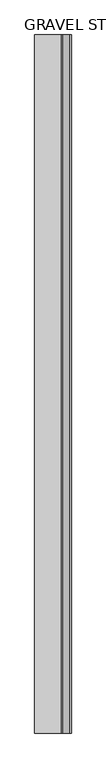
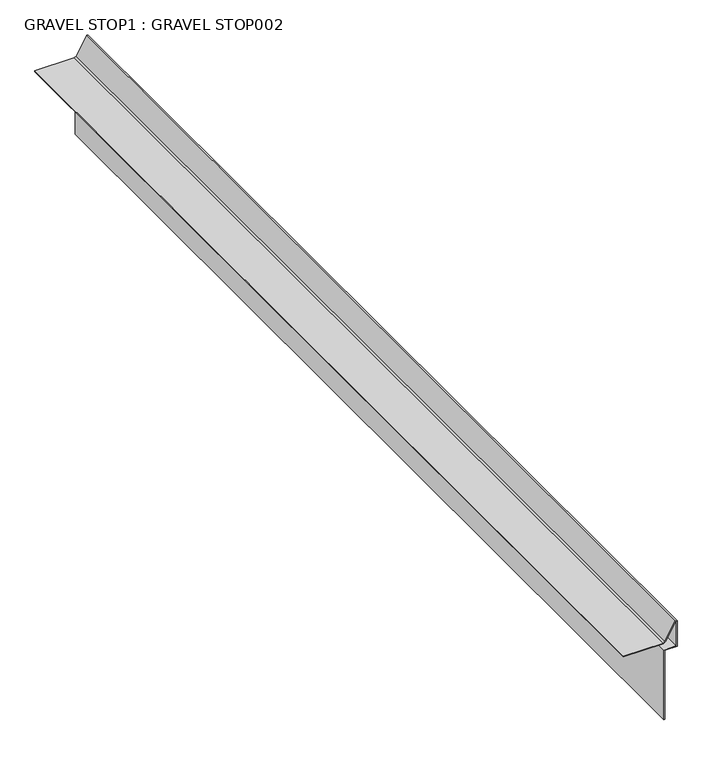
"""IFC4 building model written with IfcOpenShell, lengths in millimetres: proxy geometry, GRAVEL STOP1 : GRAVEL STOP002."""

import ifcopenshell
import ifcopenshell.guid

model = None  # the IFC model being written
_history = None  # IfcOwnerHistory: only IFC2X3 demands one
_inside = {}  # id of a spatial element -> (the spatial element, [elements in it])
_under = {}  # id of a project, library or spatial element -> (it, [spatial elements below it])
_declared = {}  # id of a project -> (the project, [libraries it declares])
_typed = {}  # id of a type object -> (the type object, [elements of that type])
_made_of = {}  # id of a material, layer set ... -> (it, [elements and type objects made of it])


def new_model(schema):
    """Start an empty IFC model of exactly this schema.

    Asked for "IFC4X3", IfcOpenShell would pick the latest addendum, in which some entities
    have other attributes; the version numbers below select the first issue.
    IFC2X3 requires an IfcOwnerHistory on every rooted entity: one is made here for all.
    """
    global model, _history
    if schema == "IFC4X3":
        model = ifcopenshell.file(schema_version=(4, 3, 0, 0))
    else:
        model = ifcopenshell.file(schema=schema)
    _inside.clear()
    _under.clear()
    _declared.clear()
    _typed.clear()
    _made_of.clear()
    _history = None
    if model.schema == "IFC2X3":
        org = make("IfcOrganization", Name="unknown")
        user = make(
            "IfcPersonAndOrganization",
            ThePerson=make("IfcPerson", FamilyName="unknown"),
            TheOrganization=org,
        )
        app = make(
            "IfcApplication",
            ApplicationDeveloper=org,
            Version="unknown",
            ApplicationFullName="unknown",
            ApplicationIdentifier="unknown",
        )
        _history = make(
            "IfcOwnerHistory",
            OwningUser=user,
            OwningApplication=app,
            ChangeAction="ADDED",
            CreationDate=0,
        )
    return model


def make(cls, **values):
    """One entity of the class cls with the attributes given. An attribute that is None is left unset."""
    return model.create_entity(
        cls, **{name: value for name, value in values.items() if value is not None}
    )


def rooted(cls, **values):
    """An entity with a GlobalId (a new one), such as an element, a storey or a relation."""
    return make(cls, GlobalId=ifcopenshell.guid.new(), OwnerHistory=_history, **values)


def si_unit(unit_type, name, prefix=None):
    """IfcSIUnit, for example si_unit("LENGTHUNIT", "METRE", prefix="MILLI")."""
    return make("IfcSIUnit", UnitType=unit_type, Prefix=prefix, Name=name)


def assignment(units):
    """IfcUnitAssignment: the units of a project."""
    return None if units is None else make("IfcUnitAssignment", Units=units)


def point(xyz):
    """IfcCartesianPoint."""
    return None if xyz is None else make("IfcCartesianPoint", Coordinates=xyz)


def direction(xyz):
    """IfcDirection."""
    return None if xyz is None else make("IfcDirection", DirectionRatios=xyz)


def frame(location, z_axis=None, x_axis=None):
    """IfcAxis2Placement3D, a coordinate frame: its origin and axes. An axis left out is left unset."""
    return make(
        "IfcAxis2Placement3D",
        Location=point(location),
        Axis=direction(z_axis),
        RefDirection=direction(x_axis),
    )


def origin():
    """The frame at (0, 0, 0) with its axes left unset."""
    return frame((0.0, 0.0, 0.0))


def place(relative_to, where):
    """IfcLocalPlacement: puts the frame where relative to a parent placement (None: the world)."""
    return make(
        "IfcLocalPlacement", PlacementRelTo=relative_to, RelativePlacement=where
    )


def context(
    kind, dimensions, precision=None, world=None, true_north=None, identifier=None
):
    """IfcGeometricRepresentationContext, for example the 3D "Model" context."""
    return make(
        "IfcGeometricRepresentationContext",
        ContextIdentifier=identifier,
        ContextType=kind,
        CoordinateSpaceDimension=dimensions,
        Precision=precision,
        WorldCoordinateSystem=world,
        TrueNorth=true_north,
    )


def project(units=None, contexts=None):
    """IfcProject with its units and contexts."""
    return rooted(
        "IfcProject",
        Name="project",
        RepresentationContexts=contexts,
        UnitsInContext=assignment(units),
    )


def spatial(cls, under=None, at=None, **own):
    """A site, building, storey or space (cls), placed at a placement, below another one or the project."""
    s = rooted(cls, ObjectPlacement=at, **own)
    if under is not None:
        _under.setdefault(under.id(), (under, []))[1].append(s)
    return s


def polyline(points):
    """IfcPolyline through the points."""
    return make("IfcPolyline", Points=[point(p) for p in points])


def outline(outer, holes=None, kind="AREA"):
    """IfcArbitraryClosedProfileDef: a profile drawn as a closed curve; with holes, ...WithVoids."""
    if holes is None:
        return make("IfcArbitraryClosedProfileDef", ProfileType=kind, OuterCurve=outer)
    return make(
        "IfcArbitraryProfileDefWithVoids",
        ProfileType=kind,
        OuterCurve=outer,
        InnerCurves=holes,
    )


def extrude(swept, where, along, depth):
    """IfcExtrudedAreaSolid: the profile swept, set in the frame where, extruded along a direction by depth."""
    return make(
        "IfcExtrudedAreaSolid",
        SweptArea=swept,
        Position=where,
        ExtrudedDirection=direction(along),
        Depth=depth,
    )


def shape(context_of_items, identifier, shape_type, items):
    """IfcShapeRepresentation: the items that make up one representation, for example the "Body"."""
    return make(
        "IfcShapeRepresentation",
        ContextOfItems=context_of_items,
        RepresentationIdentifier=identifier,
        RepresentationType=shape_type,
        Items=items,
    )


def source(mapping_origin, context_of_items, identifier, shape_type, items):
    """IfcRepresentationMap: a shape defined once, which mapped items show again and again."""
    return make(
        "IfcRepresentationMap",
        MappingOrigin=mapping_origin,
        MappedRepresentation=shape(context_of_items, identifier, shape_type, items),
    )


def transform(
    local_origin,
    x_axis=None,
    y_axis=None,
    z_axis=None,
    scale=None,
    scale2=None,
    scale3=None,
    uniform=True,
):
    """IfcCartesianTransformationOperator3D, or its non-uniform kind. x_axis, y_axis, z_axis: its Axis1, 2, 3."""
    if uniform:
        return make(
            "IfcCartesianTransformationOperator3D",
            Axis1=direction(x_axis),
            Axis2=direction(y_axis),
            LocalOrigin=point(local_origin),
            Scale=scale,
            Axis3=direction(z_axis),
        )
    return make(
        "IfcCartesianTransformationOperator3DnonUniform",
        Axis1=direction(x_axis),
        Axis2=direction(y_axis),
        LocalOrigin=point(local_origin),
        Scale=scale,
        Axis3=direction(z_axis),
        Scale2=scale2,
        Scale3=scale3,
    )


def mapped(mapping_source, mapping_target):
    """IfcMappedItem: shows the shape of a source again, moved by a transform."""
    return make(
        "IfcMappedItem", MappingSource=mapping_source, MappingTarget=mapping_target
    )


def made_of(thing, what):
    """Note that an element or type object is made of a material, layer set ...; save() writes the relation."""
    if what is not None:
        _made_of.setdefault(what.id(), (what, []))[1].append(thing)
    return thing


def element(
    cls,
    number,
    at=None,
    inside=None,
    cuts=None,
    type_object=None,
    material=None,
    context=None,
    identifier="Body",
    shape_type=None,
    held_by="IfcProductDefinitionShape",
    body=None,
    shapes=None,
    **own,
):
    """One element of the class cls, such as IfcWall. Its Tag is "e" and its number.

    at: its placement. inside: the storey or other place that contains it. cuts: it is an
    opening in that element (IfcRelVoidsElement). A single representation is given by context,
    identifier, shape_type and body (its items); several are given by shapes. held_by: the class
    of the entity that holds the representations. save() writes the other relations.
    """
    e = rooted(cls, Tag="e%d" % number, ObjectPlacement=at, **own)
    if body is not None:
        shapes = [shape(context, identifier, shape_type, body)]
    if shapes is not None:
        e.Representation = make(held_by, Representations=shapes)
    if inside is not None:
        _inside.setdefault(inside.id(), (inside, []))[1].append(e)
    if cuts is not None:
        rooted(
            "IfcRelVoidsElement", RelatingBuildingElement=cuts, RelatedOpeningElement=e
        )
    if type_object is not None:
        _typed.setdefault(type_object.id(), (type_object, []))[1].append(e)
    return made_of(e, material)


def aggregate(whole, parts):
    """IfcRelAggregates: a whole, such as a stair, and the parts it consists of."""
    return rooted("IfcRelAggregates", RelatingObject=whole, RelatedObjects=parts)


def save(model, path):
    """Write the relations noted so far, then the file.

    IfcRelAggregates (storeys below a building ...), IfcRelContainedInSpatialStructure (elements
    in a storey), IfcRelDefinesByType, IfcRelAssociatesMaterial and IfcRelDeclares: one each for
    every whole, place, type object, material and project.
    """
    for whole, parts in _under.values():
        aggregate(whole, parts)
    for where, things in _inside.values():
        rooted(
            "IfcRelContainedInSpatialStructure",
            RelatedElements=things,
            RelatingStructure=where,
        )
    for kind, things in _typed.values():
        rooted("IfcRelDefinesByType", RelatedObjects=things, RelatingType=kind)
    for what, things in _made_of.values():
        rooted("IfcRelAssociatesMaterial", RelatedObjects=things, RelatingMaterial=what)
    for by, libraries in _declared.values():
        rooted("IfcRelDeclares", RelatingContext=by, RelatedDefinitions=libraries)
    model.write(path)


def gravel_stop1_gravel_stop002_7041c615(model_context):
    return source(origin(), model_context, "Body", "SweptSolid", [
        extrude(outline(polyline([(40295.3431515, -4364.7039765), (40259.5408757, -4385.3744301), (40257.3744784, -4389.1267403), (40257.3744784, -4466.584647), (40255.9633674, -4466.584647), (40255.9633674, -4388.7486343), (40258.5078708, -4384.3414252), (40293.699878, -4364.0233103), (40293.447969, -4363.0831732), (40242.3744784, -4363.0831732), (40242.3744784, -4387.4229108), (40097.9858473, -4387.4229108), (40097.9858473, -4386.0117998), (40240.9633674, -4386.0117998), (40240.9633674, -4361.6720622), (40294.5307525, -4361.6720622), (40295.3431515, -4364.7039765)])), frame((0.0, -1052.8906573, 0.0), z_axis=(0.0, 1.0, 0.0), x_axis=(0.0, 0.0, 1.0)), (0.0, 0.0, 1.0), 2000.25),
    ])


if __name__ == "__main__":
    model = new_model("IFC4")
    model_context = context("Model", 3, world=origin())
    ifc_project = project(units=[si_unit("LENGTHUNIT", "METRE", prefix="MILLI")], contexts=[model_context])
    site = spatial("IfcSite", under=ifc_project)
    building = spatial("IfcBuilding", under=site)
    placement = place(None, origin())
    gravel_stop1_gravel_stop002_shape = gravel_stop1_gravel_stop002_7041c615(model_context)
    element("IfcBuildingElementProxy", 1, Name="GRAVEL STOP1 : GRAVEL STOP002", ObjectType="GRAVEL STOP1 : GRAVEL STOP002", at=placement, inside=building, context=model_context, shape_type="MappedRepresentation", body=[
        mapped(gravel_stop1_gravel_stop002_shape, transform((0.0, 0.0, 0.0), x_axis=(1.0, 0.0, 0.0), y_axis=(0.0, 1.0, 0.0), z_axis=(0.0, 0.0, 1.0))),
    ])
    save(model, "model.ifc")

# Revit data of these elements
# Type "GRAVEL STOP1 : GRAVEL STOP002"
#   NameOverride = "GRAVEL STOP002"
# Element 1 (IfcBuildingElementProxy, "GRAVEL STOP1 : GRAVEL STOP002")
#   Materials on its faces: "GRAVEL STOP REQUIRED WITH GRAVEL SURFACE SYSTEMS"
# Materials
#   "GRAVEL STOP REQUIRED WITH GRAVEL SURFACE SYSTEMS": class "Unassigned", colour RGB 170 170 127, transparency 0, Cost = 0
